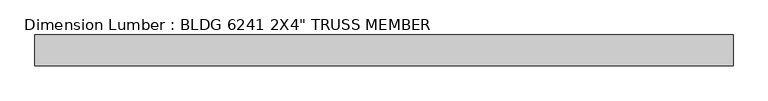
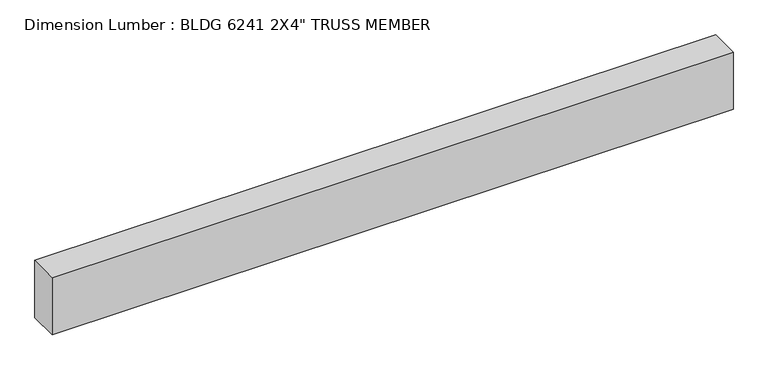
"""IFC4 building model written with IfcOpenShell, lengths in millimetres: beam geometry."""

from ifc_helpers import new_model, si_unit, frame, origin, place, context, project, spatial, polyline, outline, extrude, source, transform, mapped, element, save


def beam_38e3f9e5(model_context):
    return source(origin(), model_context, "Body", "SweptSolid", [
        extrude(outline(polyline([(595.8662636, -25.4), (-548.2789755, -25.4), (-548.2789755, 25.4), (595.8662636, 25.4), (595.8662636, -25.4)])), frame((0.0, 0.0, -50.8), z_axis=(0.0, 0.0, 1.0), x_axis=(1.0, 0.0, 0.0)), (0.0, 0.0, 1.0), 101.6),
    ])


if __name__ == "__main__":
    model = new_model("IFC4")
    model_context = context("Model", 3, world=origin())
    ifc_project = project(units=[si_unit("LENGTHUNIT", "METRE", prefix="MILLI")], contexts=[model_context])
    site = spatial("IfcSite", under=ifc_project)
    building = spatial("IfcBuilding", under=site)
    placement = place(None, origin())
    beam_shape = beam_38e3f9e5(model_context)
    element("IfcBeam", 1, ObjectType="Dimension Lumber : BLDG 6241 2X4\" TRUSS MEMBER", at=placement, inside=building, context=model_context, shape_type="MappedRepresentation", body=[
        mapped(beam_shape, transform((0.0, 0.0, 0.0), x_axis=(1.0, 0.0, 0.0), y_axis=(0.0, 1.0, 0.0), z_axis=(0.0, 0.0, 1.0))),
    ])
    save(model, "model.ifc")

# Revit data of these elements
# Type "Dimension Lumber : BLDG 6241 2X4\" TRUSS MEMBER"
#   Assembly Code = "B10"
#   A = 0.273472 SF
#   Length [instance default] = 5' - 0"
#   b = 0' - 2"
#   d = 0' - 4"
#   Structural Material [instance default] = Softwood, Lumber
# Element 1 (IfcBeam, "Dimension Lumber : BLDG 6241 2X4\" TRUSS MEMBER")
#   Materials on its faces: "Softwood, Lumber"
# Materials
#   "Softwood, Lumber": class "Wood", colour RGB 223 192 134, transparency 0, Description = "Pinus Echinata", Cost = 0
